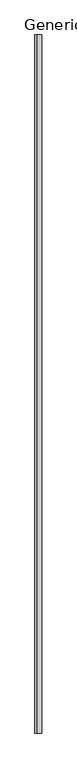
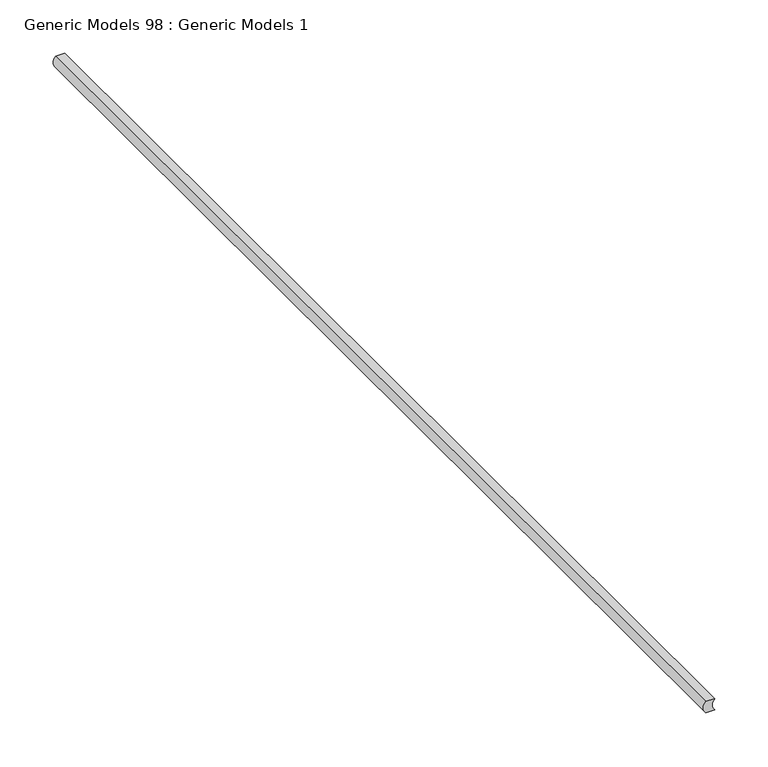
"""IFC4 building model written with IfcOpenShell, lengths in millimetres: proxy geometry, Generic Models 98 : Generic Models 1."""

import ifcopenshell
import ifcopenshell.guid

model = None  # the IFC model being written
_history = None  # IfcOwnerHistory: only IFC2X3 demands one
_inside = {}  # id of a spatial element -> (the spatial element, [elements in it])
_under = {}  # id of a project, library or spatial element -> (it, [spatial elements below it])
_declared = {}  # id of a project -> (the project, [libraries it declares])
_typed = {}  # id of a type object -> (the type object, [elements of that type])
_made_of = {}  # id of a material, layer set ... -> (it, [elements and type objects made of it])


def new_model(schema):
    """Start an empty IFC model of exactly this schema.

    Asked for "IFC4X3", IfcOpenShell would pick the latest addendum, in which some entities
    have other attributes; the version numbers below select the first issue.
    IFC2X3 requires an IfcOwnerHistory on every rooted entity: one is made here for all.
    """
    global model, _history
    if schema == "IFC4X3":
        model = ifcopenshell.file(schema_version=(4, 3, 0, 0))
    else:
        model = ifcopenshell.file(schema=schema)
    _inside.clear()
    _under.clear()
    _declared.clear()
    _typed.clear()
    _made_of.clear()
    _history = None
    if model.schema == "IFC2X3":
        org = make("IfcOrganization", Name="unknown")
        user = make(
            "IfcPersonAndOrganization",
            ThePerson=make("IfcPerson", FamilyName="unknown"),
            TheOrganization=org,
        )
        app = make(
            "IfcApplication",
            ApplicationDeveloper=org,
            Version="unknown",
            ApplicationFullName="unknown",
            ApplicationIdentifier="unknown",
        )
        _history = make(
            "IfcOwnerHistory",
            OwningUser=user,
            OwningApplication=app,
            ChangeAction="ADDED",
            CreationDate=0,
        )
    return model


def make(cls, **values):
    """One entity of the class cls with the attributes given. An attribute that is None is left unset."""
    return model.create_entity(
        cls, **{name: value for name, value in values.items() if value is not None}
    )


def rooted(cls, **values):
    """An entity with a GlobalId (a new one), such as an element, a storey or a relation."""
    return make(cls, GlobalId=ifcopenshell.guid.new(), OwnerHistory=_history, **values)


def si_unit(unit_type, name, prefix=None):
    """IfcSIUnit, for example si_unit("LENGTHUNIT", "METRE", prefix="MILLI")."""
    return make("IfcSIUnit", UnitType=unit_type, Prefix=prefix, Name=name)


def assignment(units):
    """IfcUnitAssignment: the units of a project."""
    return None if units is None else make("IfcUnitAssignment", Units=units)


def point(xyz):
    """IfcCartesianPoint."""
    return None if xyz is None else make("IfcCartesianPoint", Coordinates=xyz)


def direction(xyz):
    """IfcDirection."""
    return None if xyz is None else make("IfcDirection", DirectionRatios=xyz)


def frame(location, z_axis=None, x_axis=None):
    """IfcAxis2Placement3D, a coordinate frame: its origin and axes. An axis left out is left unset."""
    return make(
        "IfcAxis2Placement3D",
        Location=point(location),
        Axis=direction(z_axis),
        RefDirection=direction(x_axis),
    )


def frame_2d(location, x_axis=None):
    """IfcAxis2Placement2D, a coordinate frame in the plane: its origin and x axis."""
    return make(
        "IfcAxis2Placement2D", Location=point(location), RefDirection=direction(x_axis)
    )


def origin():
    """The frame at (0, 0, 0) with its axes left unset."""
    return frame((0.0, 0.0, 0.0))


def place(relative_to, where):
    """IfcLocalPlacement: puts the frame where relative to a parent placement (None: the world)."""
    return make(
        "IfcLocalPlacement", PlacementRelTo=relative_to, RelativePlacement=where
    )


def context(
    kind, dimensions, precision=None, world=None, true_north=None, identifier=None
):
    """IfcGeometricRepresentationContext, for example the 3D "Model" context."""
    return make(
        "IfcGeometricRepresentationContext",
        ContextIdentifier=identifier,
        ContextType=kind,
        CoordinateSpaceDimension=dimensions,
        Precision=precision,
        WorldCoordinateSystem=world,
        TrueNorth=true_north,
    )


def project(units=None, contexts=None):
    """IfcProject with its units and contexts."""
    return rooted(
        "IfcProject",
        Name="project",
        RepresentationContexts=contexts,
        UnitsInContext=assignment(units),
    )


def spatial(cls, under=None, at=None, **own):
    """A site, building, storey or space (cls), placed at a placement, below another one or the project."""
    s = rooted(cls, ObjectPlacement=at, **own)
    if under is not None:
        _under.setdefault(under.id(), (under, []))[1].append(s)
    return s


def polyline(points):
    """IfcPolyline through the points."""
    return make("IfcPolyline", Points=[point(p) for p in points])


def circle_curve(where, radius):
    """IfcCircle in the frame where."""
    return make("IfcCircle", Position=where, Radius=radius)


def trimmed(basis, trim1, trim2, sense, master):
    """IfcTrimmedCurve: the piece of a basis curve between two trims."""
    return make(
        "IfcTrimmedCurve",
        BasisCurve=basis,
        Trim1=trim1,
        Trim2=trim2,
        SenseAgreement=sense,
        MasterRepresentation=master,
    )


def segment(curve, same_sense, transition):
    """IfcCompositeCurveSegment."""
    return make(
        "IfcCompositeCurveSegment",
        Transition=transition,
        SameSense=same_sense,
        ParentCurve=curve,
    )


def composite_curve(segments, self_intersect=None):
    """IfcCompositeCurve: segments joined end to end."""
    return make("IfcCompositeCurve", Segments=segments, SelfIntersect=self_intersect)


def outline(outer, holes=None, kind="AREA"):
    """IfcArbitraryClosedProfileDef: a profile drawn as a closed curve; with holes, ...WithVoids."""
    if holes is None:
        return make("IfcArbitraryClosedProfileDef", ProfileType=kind, OuterCurve=outer)
    return make(
        "IfcArbitraryProfileDefWithVoids",
        ProfileType=kind,
        OuterCurve=outer,
        InnerCurves=holes,
    )


def extrude(swept, where, along, depth):
    """IfcExtrudedAreaSolid: the profile swept, set in the frame where, extruded along a direction by depth."""
    return make(
        "IfcExtrudedAreaSolid",
        SweptArea=swept,
        Position=where,
        ExtrudedDirection=direction(along),
        Depth=depth,
    )


def shape(context_of_items, identifier, shape_type, items):
    """IfcShapeRepresentation: the items that make up one representation, for example the "Body"."""
    return make(
        "IfcShapeRepresentation",
        ContextOfItems=context_of_items,
        RepresentationIdentifier=identifier,
        RepresentationType=shape_type,
        Items=items,
    )


def source(mapping_origin, context_of_items, identifier, shape_type, items):
    """IfcRepresentationMap: a shape defined once, which mapped items show again and again."""
    return make(
        "IfcRepresentationMap",
        MappingOrigin=mapping_origin,
        MappedRepresentation=shape(context_of_items, identifier, shape_type, items),
    )


def transform(
    local_origin,
    x_axis=None,
    y_axis=None,
    z_axis=None,
    scale=None,
    scale2=None,
    scale3=None,
    uniform=True,
):
    """IfcCartesianTransformationOperator3D, or its non-uniform kind. x_axis, y_axis, z_axis: its Axis1, 2, 3."""
    if uniform:
        return make(
            "IfcCartesianTransformationOperator3D",
            Axis1=direction(x_axis),
            Axis2=direction(y_axis),
            LocalOrigin=point(local_origin),
            Scale=scale,
            Axis3=direction(z_axis),
        )
    return make(
        "IfcCartesianTransformationOperator3DnonUniform",
        Axis1=direction(x_axis),
        Axis2=direction(y_axis),
        LocalOrigin=point(local_origin),
        Scale=scale,
        Axis3=direction(z_axis),
        Scale2=scale2,
        Scale3=scale3,
    )


def mapped(mapping_source, mapping_target):
    """IfcMappedItem: shows the shape of a source again, moved by a transform."""
    return make(
        "IfcMappedItem", MappingSource=mapping_source, MappingTarget=mapping_target
    )


def made_of(thing, what):
    """Note that an element or type object is made of a material, layer set ...; save() writes the relation."""
    if what is not None:
        _made_of.setdefault(what.id(), (what, []))[1].append(thing)
    return thing


def element(
    cls,
    number,
    at=None,
    inside=None,
    cuts=None,
    type_object=None,
    material=None,
    context=None,
    identifier="Body",
    shape_type=None,
    held_by="IfcProductDefinitionShape",
    body=None,
    shapes=None,
    **own,
):
    """One element of the class cls, such as IfcWall. Its Tag is "e" and its number.

    at: its placement. inside: the storey or other place that contains it. cuts: it is an
    opening in that element (IfcRelVoidsElement). A single representation is given by context,
    identifier, shape_type and body (its items); several are given by shapes. held_by: the class
    of the entity that holds the representations. save() writes the other relations.
    """
    e = rooted(cls, Tag="e%d" % number, ObjectPlacement=at, **own)
    if body is not None:
        shapes = [shape(context, identifier, shape_type, body)]
    if shapes is not None:
        e.Representation = make(held_by, Representations=shapes)
    if inside is not None:
        _inside.setdefault(inside.id(), (inside, []))[1].append(e)
    if cuts is not None:
        rooted(
            "IfcRelVoidsElement", RelatingBuildingElement=cuts, RelatedOpeningElement=e
        )
    if type_object is not None:
        _typed.setdefault(type_object.id(), (type_object, []))[1].append(e)
    return made_of(e, material)


def aggregate(whole, parts):
    """IfcRelAggregates: a whole, such as a stair, and the parts it consists of."""
    return rooted("IfcRelAggregates", RelatingObject=whole, RelatedObjects=parts)


def save(model, path):
    """Write the relations noted so far, then the file.

    IfcRelAggregates (storeys below a building ...), IfcRelContainedInSpatialStructure (elements
    in a storey), IfcRelDefinesByType, IfcRelAssociatesMaterial and IfcRelDeclares: one each for
    every whole, place, type object, material and project.
    """
    for whole, parts in _under.values():
        aggregate(whole, parts)
    for where, things in _inside.values():
        rooted(
            "IfcRelContainedInSpatialStructure",
            RelatedElements=things,
            RelatingStructure=where,
        )
    for kind, things in _typed.values():
        rooted("IfcRelDefinesByType", RelatedObjects=things, RelatingType=kind)
    for what, things in _made_of.values():
        rooted("IfcRelAssociatesMaterial", RelatedObjects=things, RelatingMaterial=what)
    for by, libraries in _declared.values():
        rooted("IfcRelDeclares", RelatingContext=by, RelatedDefinitions=libraries)
    model.write(path)


def generic_models_98_generic_models_1_0e24db6d(model_context):
    return source(origin(), model_context, "Body", "SweptSolid", [
        extrude(outline(composite_curve([segment(trimmed(circle_curve(frame_2d((300.6766124, 49824.0226449)), 8.620055), [point((294.3266124, 49818.1931639))], [point((307.0266124, 49818.1931639))], True, "CARTESIAN"), True, "CONTINUOUS"), segment(polyline([(307.0266124, 49818.1931639), (307.0266124, 49808.6681639)]), True, "CONTINUOUS"), segment(trimmed(circle_curve(frame_2d((300.6766124, 49814.4976449)), 8.620055), [point((307.0266124, 49808.6681639))], [point((294.3266124, 49808.6681639))], False, "CARTESIAN"), True, "CONTINUOUS"), segment(polyline([(294.3266124, 49808.6681639), (294.3266124, 49818.1931639)]), True, "CONTINUOUS")], self_intersect=False)), frame((0.0, 0.0, 0.0), z_axis=(0.0, 1.0, 0.0), x_axis=(0.0, 0.0, 1.0)), (0.0, 0.0, 1.0), 1219.2),
    ])


if __name__ == "__main__":
    model = new_model("IFC4")
    model_context = context("Model", 3, world=origin())
    ifc_project = project(units=[si_unit("LENGTHUNIT", "METRE", prefix="MILLI")], contexts=[model_context])
    site = spatial("IfcSite", under=ifc_project)
    building = spatial("IfcBuilding", under=site)
    placement = place(None, origin())
    generic_models_98_generic_models_1_shape = generic_models_98_generic_models_1_0e24db6d(model_context)
    element("IfcBuildingElementProxy", 1, Name="Generic Models 98 : Generic Models 1", ObjectType="Generic Models 98 : Generic Models 1", at=placement, inside=building, context=model_context, shape_type="MappedRepresentation", body=[
        mapped(generic_models_98_generic_models_1_shape, transform((0.0, 0.0, 0.0), x_axis=(1.0, 0.0, 0.0), y_axis=(0.0, 1.0, 0.0), z_axis=(0.0, 0.0, 1.0))),
    ])
    save(model, "model.ifc")

# Revit data of these elements
# Element 1 (IfcBuildingElementProxy, "Generic Models 98 : Generic Models 1")
#   Materials on its faces: "SEALANT (W/ BACKER ROD IF NECESSARY)"
# Materials
#   "SEALANT (W/ BACKER ROD IF NECESSARY)": class "Unassigned", colour RGB 120 120 120, transparency 0, Cost = 0
